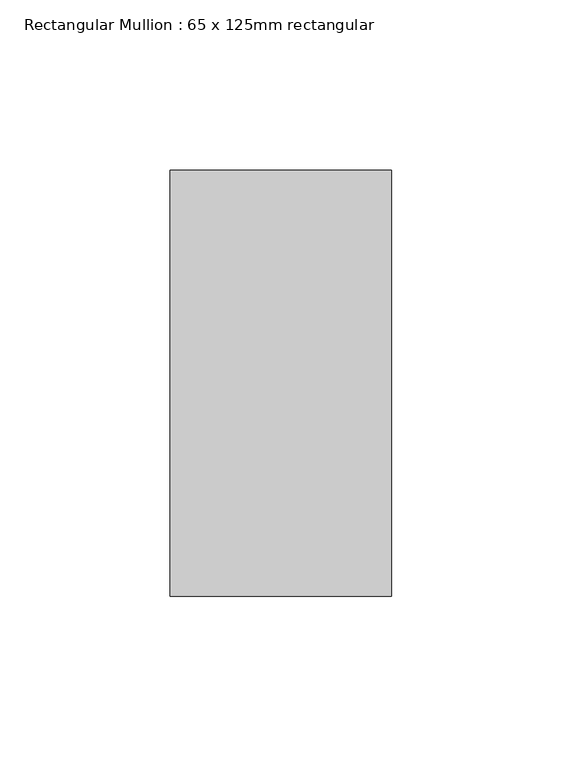
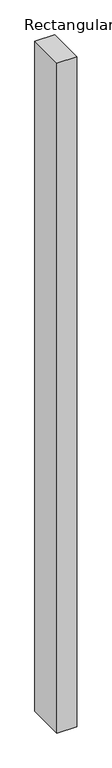
"""IFC4 building model written with IfcOpenShell, lengths in millimetres: member geometry, Rectangular Mullion : 65 x 125mm rectangular."""

from ifc_helpers import new_model, si_unit, frame, origin, place, context, project, spatial, polyline, outline, extrude, source, transform, mapped, element, save


def rectangular_mullion_65_x_125mm_rectangular_eddbc5d6(model_context):
    return source(origin(), model_context, "Body", "SweptSolid", [
        extrude(outline(polyline([(0.0, 62.5), (0.0, -62.5), (-65.0, -62.5), (-65.0, 62.5), (0.0, 62.5)])), frame((0.0, 0.0, -2323.142254), z_axis=(0.0, 0.0, 1.0), x_axis=(1.0, 0.0, 0.0)), (0.0, 0.0, 1.0), 2323.142254),
    ])


if __name__ == "__main__":
    model = new_model("IFC4")
    model_context = context("Model", 3, world=origin())
    ifc_project = project(units=[si_unit("LENGTHUNIT", "METRE", prefix="MILLI")], contexts=[model_context])
    site = spatial("IfcSite", under=ifc_project)
    building = spatial("IfcBuilding", under=site)
    placement = place(None, origin())
    rectangular_mullion_65_x_125mm_rectangular_shape = rectangular_mullion_65_x_125mm_rectangular_eddbc5d6(model_context)
    element("IfcMember", 1, ObjectType="Rectangular Mullion : 65 x 125mm rectangular", at=placement, inside=building, context=model_context, shape_type="MappedRepresentation", body=[
        mapped(rectangular_mullion_65_x_125mm_rectangular_shape, transform((0.0, 0.0, 0.0), x_axis=(1.0, 0.0, 0.0), y_axis=(0.0, 1.0, 0.0), z_axis=(0.0, 0.0, 1.0))),
    ])
    save(model, "model.ifc")

# Revit data of these elements
# Type "Rectangular Mullion : 65 x 125mm rectangular"
#   built-in parameter 1007304 = 0.410105 (stored number, unit not read)
#   built-in parameter 1007301 = 0.106627 (stored number, unit not read)
#   built-in parameter 1007300 = 0.106627 (stored number, unit not read)
# Element 1 (IfcMember, "Rectangular Mullion : 65 x 125mm rectangular")
#   Materials on its faces: "Aluminum"
# Materials
#   "Aluminum": class "Metal", colour RGB 244 245 246, transparency 0, Description = "Aluminum 6061", Cost = 0
